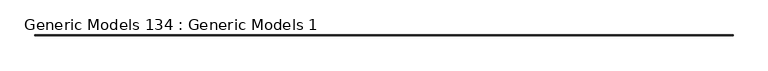
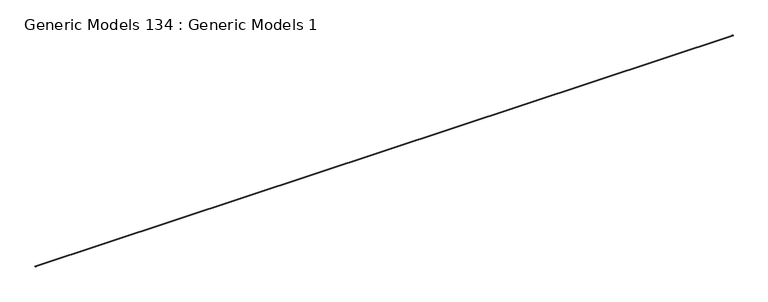
"""IFC4 building model written with IfcOpenShell, lengths in millimetres: proxy geometry, Generic Models 134 : Generic Models 1."""

from ifc_helpers import new_model, si_unit, point, frame, origin, place, context, project, spatial, polyline, circle_curve, ellipse_curve, trimmed, source, transform, mapped, element, save
from ifc_brep_helpers import plane_surface, cylinder_surface, revolved_surface, extruded_surface, advanced_brep


def generic_models_134_generic_models_1_a6a1a120(model_context):
    return source(origin(), model_context, "Body", "AdvancedBrep", [
        advanced_brep(
        [(2853.9658099, 13215.1765847, 129231.5872789), (2853.9658099, 13215.1765847, 129241.1122789), (2853.9658099, 13219.9390847, 129241.1122789), (2853.9658099, 13221.3667236, 129239.206291), (2853.9658099, 13221.3667236, 129233.4932667), (2853.9658099, 13219.9390847, 129231.5872789), (21903.9658099, 13215.1765847, 129231.5872789), (21903.9658099, 13219.9390847, 129231.5872789), (21903.9658099, 13221.3667236, 129233.4932667), (21903.9658099, 13221.3667236, 129239.206291), (21903.9658099, 13219.9390847, 129241.1122789), (21903.9658099, 13215.1765847, 129241.1122789)],
        [
            (0, 1, circle_curve(frame((2853.9658099, 13210.8044739, 129236.3497789), z_axis=(1.0, 0.0, 0.0), x_axis=(0.0, 0.0, -1.0)), 6.4650413)),
            (1, 2),
            (2, 3, circle_curve(frame((2853.9658099, 13215.5669739, 129236.3497789), z_axis=(-1.0, 0.0, 0.0), x_axis=(0.0, 0.0, -1.0)), 6.4650413)),
            (3, 4, ellipse_curve(frame((2853.9658099, 13227.0828347, 129236.3497789), z_axis=(-1.0, 0.0, 0.0), x_axis=(0.0, -1.0, 0.0)), 7.14375, 4.7625)),
            (4, 5, circle_curve(frame((2853.9658099, 13215.5669739, 129236.3497789), z_axis=(-1.0, 0.0, 0.0), x_axis=(0.0, 0.0, -1.0)), 6.4650413)),
            (5, 0),
            (6, 7),
            (7, 8, circle_curve(frame((21903.9658099, 13215.5669739, 129236.3497789), z_axis=(1.0, 0.0, 0.0), x_axis=(0.0, 0.0, -1.0)), 6.4650413)),
            (8, 9, ellipse_curve(frame((21903.9658099, 13227.0828347, 129236.3497789), z_axis=(1.0, 0.0, 0.0), x_axis=(0.0, -1.0, 0.0)), 7.14375, 4.7625)),
            (9, 10, circle_curve(frame((21903.9658099, 13215.5669739, 129236.3497789), z_axis=(1.0, 0.0, 0.0), x_axis=(0.0, 0.0, -1.0)), 6.4650413)),
            (10, 11),
            (11, 6, circle_curve(frame((21903.9658099, 13210.8044739, 129236.3497789), z_axis=(-1.0, 0.0, 0.0), x_axis=(0.0, 0.0, -1.0)), 6.4650413)),
            (3, 9),
            (8, 4),
            (0, 6),
            (11, 1),
            (10, 2),
            (7, 5),
        ],
        [
            plane_surface(frame((2853.9658099, 13215.1765847, 129241.1122789), z_axis=(-1.0, 0.0, 0.0), x_axis=(0.0, -1.0, 0.0))),
            plane_surface(frame((21903.9658099, 13215.1765847, 129241.1122789), z_axis=(1.0, 0.0, 0.0), x_axis=(0.0, -1.0, 0.0))),
            extruded_surface(trimmed(ellipse_curve(frame((21903.9658099, 13227.0828347, 129236.3497789), z_axis=(-1.0, 0.0, 0.0), x_axis=(0.0, -1.0, 0.0)), 7.14375, 4.7625), [point((21903.9658099, 13221.3667236, 129239.206291))], [point((21903.9658099, 13221.3667236, 129233.4932667))], True, "CARTESIAN"), (-19050.0, 0.0, 0.0), 19050.0),
            revolved_surface(polyline([(21903.9658099, 13210.8044739, 129229.88473759999), (2853.9658099, 13210.8044739, 129229.88473759999)]), (2853.9658099, 13210.8044739, 129236.3497789), (1.0, 0.0, 0.0)),
            plane_surface(frame((2853.9658099, 13215.1765847, 129241.1122789), z_axis=(0.0, 0.0, 1.0), x_axis=(1.0, 0.0, 0.0))),
            cylinder_surface(frame((2853.9658099, 13215.5669739, 129236.3497789), z_axis=(-1.0, 0.0, 0.0), x_axis=(0.0, 0.0, -1.0)), 6.4650413),
            plane_surface(frame((2853.9658099, 13219.9390847, 129231.5872789), z_axis=(0.0, 0.0, -1.0), x_axis=(1.0, 0.0, 0.0))),
        ],
        [
            (0, [[1, 2, 3, 4, 5, 6]]),
            (1, [[7, 8, 9, 10, 11, 12]]),
            (2, [[-4, 13, -9, 14]]),
            (3, [[-1, 15, -12, 16]]),
            (4, [[-2, -16, -11, 17]]),
            (5, [[-3, -17, -10, -13]]),
            (5, [[-5, -14, -8, 18]]),
            (6, [[-6, -18, -7, -15]]),
        ],
    ),
    ])


if __name__ == "__main__":
    model = new_model("IFC4")
    model_context = context("Model", 3, world=origin())
    ifc_project = project(units=[si_unit("LENGTHUNIT", "METRE", prefix="MILLI")], contexts=[model_context])
    site = spatial("IfcSite", under=ifc_project)
    building = spatial("IfcBuilding", under=site)
    placement = place(None, origin())
    generic_models_134_generic_models_1_shape = generic_models_134_generic_models_1_a6a1a120(model_context)
    element("IfcBuildingElementProxy", 1, Name="Generic Models 134 : Generic Models 1", ObjectType="Generic Models 134 : Generic Models 1", at=placement, inside=building, context=model_context, shape_type="MappedRepresentation", body=[
        mapped(generic_models_134_generic_models_1_shape, transform((0.0, 0.0, 0.0), x_axis=(1.0, 0.0, 0.0), y_axis=(0.0, 1.0, 0.0), z_axis=(0.0, 0.0, 1.0))),
    ])
    save(model, "model.ifc")

# Revit data of these elements
# Element 1 (IfcBuildingElementProxy, "Generic Models 134 : Generic Models 1")
#   Materials on its faces: "_SEALANT AND BACKROD, IF NEC."
# Materials
#   "_SEALANT AND BACKROD, IF NEC.": class "Generic", colour RGB 190 220 196, transparency 0, Cost = 0
